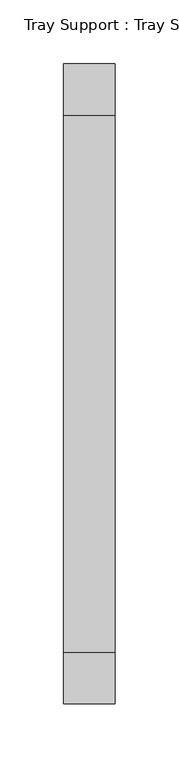
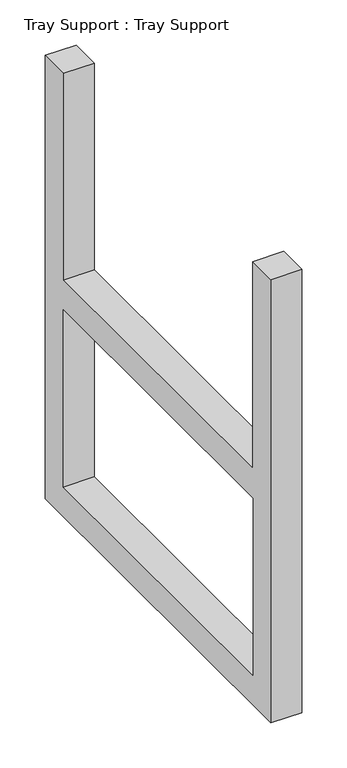
"""IFC4 building model written with IfcOpenShell, lengths in millimetres: proxy geometry, Tray Support : Tray Support."""

from ifc_helpers import new_model, si_unit, frame, origin, place, context, project, spatial, polyline, outline, extrude, source, transform, mapped, element, save


def tray_support_tray_support_8a820f0e(model_context):
    return source(origin(), model_context, "Body", "SweptSolid", [
        extrude(outline(polyline([(14077.8336064, 6254.605), (13577.8336064, 6254.605), (13577.8336064, 6854.605), (13617.8336064, 6854.605), (13617.8336064, 6574.605), (14037.8336064, 6574.605), (14037.8336064, 6854.605), (14077.8336064, 6854.605), (14077.8336064, 6254.605)]), holes=[polyline([(13617.8336064, 6294.605), (14037.8336064, 6294.605), (14037.8336064, 6534.605), (13617.8336064, 6534.605), (13617.8336064, 6294.605)])]), frame((-12977.2499534, 0.0, 0.0), z_axis=(1.0, 0.0, 0.0), x_axis=(0.0, 1.0, 0.0)), (0.0, 0.0, 1.0), 40.0),
    ])


if __name__ == "__main__":
    model = new_model("IFC4")
    model_context = context("Model", 3, world=origin())
    ifc_project = project(units=[si_unit("LENGTHUNIT", "METRE", prefix="MILLI")], contexts=[model_context])
    site = spatial("IfcSite", under=ifc_project)
    building = spatial("IfcBuilding", under=site)
    placement = place(None, origin())
    tray_support_tray_support_shape = tray_support_tray_support_8a820f0e(model_context)
    element("IfcBuildingElementProxy", 1, Name="Tray Support : Tray Support", ObjectType="Tray Support : Tray Support", at=placement, inside=building, context=model_context, shape_type="MappedRepresentation", body=[
        mapped(tray_support_tray_support_shape, transform((0.0, 0.0, 0.0), x_axis=(1.0, 0.0, 0.0), y_axis=(0.0, 1.0, 0.0), z_axis=(0.0, 0.0, 1.0))),
    ])
    save(model, "model.ifc")
